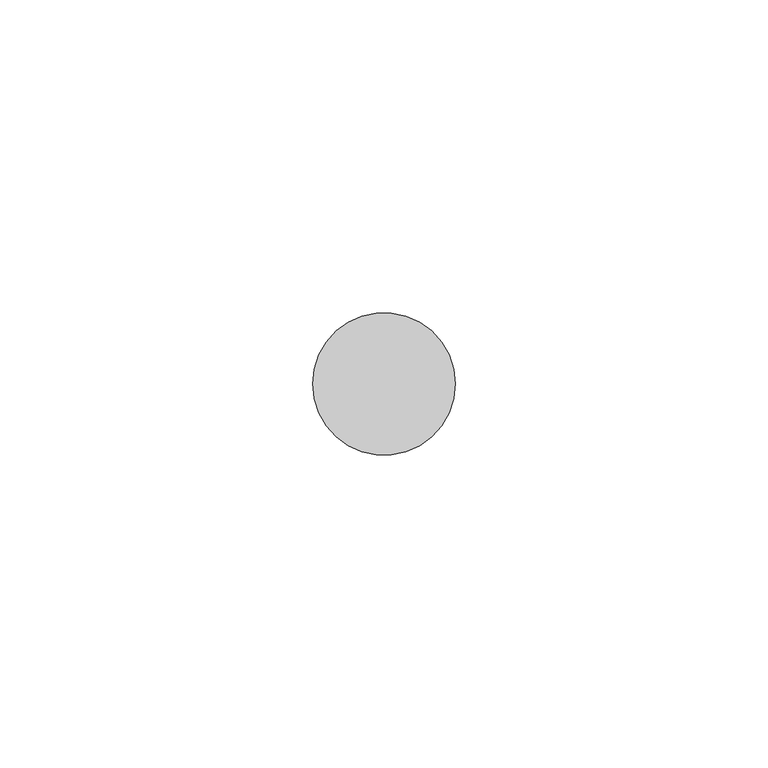
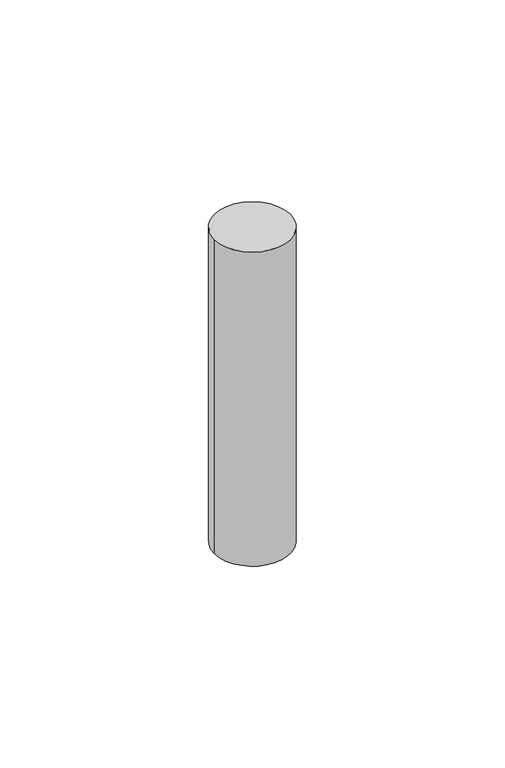
"""IFC4 building model written with IfcOpenShell, lengths in millimetres: proxy geometry, Bolt7:Bolt003:302961 : Bolt7:Bolt003:302961."""

from ifc_helpers import new_model, si_unit, point, frame, frame_2d, origin, place, context, project, spatial, circle_curve, trimmed, segment, composite_curve, outline, extrude, source, transform, mapped, element, save


def generic_models_6c568443(model_context):
    return source(origin(), model_context, "Body", "SweptSolid", [
        extrude(outline(composite_curve([segment(trimmed(circle_curve(frame_2d((12192.2703385, -1503.5124296)), 11.4045168), [point((12180.8658216, -1503.5124296))], [point((12203.6748553, -1503.5124296))], False, "CARTESIAN"), True, "CONTINUOUS"), segment(trimmed(circle_curve(frame_2d((12192.2703385, -1503.5124296)), 11.4045168), [point((12203.6748553, -1503.5124296))], [point((12180.8658216, -1503.5124296))], False, "CARTESIAN"), True, "CONTINUOUS")], self_intersect=False)), frame((0.0, 0.0, 39994.0914664), z_axis=(0.0, 0.0, 1.0), x_axis=(1.0, 0.0, 0.0)), (0.0, 0.0, 1.0), 99.5545336),
    ])


if __name__ == "__main__":
    model = new_model("IFC4")
    model_context = context("Model", 3, world=origin())
    ifc_project = project(units=[si_unit("LENGTHUNIT", "METRE", prefix="MILLI")], contexts=[model_context])
    site = spatial("IfcSite", under=ifc_project)
    building = spatial("IfcBuilding", under=site)
    placement = place(None, origin())
    generic_models_shape = generic_models_6c568443(model_context)
    element("IfcBuildingElementProxy", 1, Name="Bolt7:Bolt003:302961 : Bolt7:Bolt003:302961", ObjectType="Bolt7:Bolt003:302961 : Bolt7:Bolt003:302961", at=placement, inside=building, context=model_context, shape_type="MappedRepresentation", body=[
        mapped(generic_models_shape, transform((0.0, 0.0, 0.0), x_axis=(1.0, 0.0, 0.0), y_axis=(0.0, 1.0, 0.0), z_axis=(0.0, 0.0, 1.0))),
    ])
    save(model, "model.ifc")

# Revit data of these elements
# Type "Bolt7:Bolt003:302961 : Bolt7:Bolt003:302961"
#   NameOverride = "Bolt7:Bolt003:302961"
#   ObjectTypeOverride = "Bolt7:Bolt003"
#   Reference = "Bolt003"
#   Category = "Generic Models"
#   Tag = "302961"
# Element 1 (IfcBuildingElementProxy, "Bolt7:Bolt003:302961 : Bolt7:Bolt003:302961")
#   Materials on its faces: "BOLTS CONCEALED BY FLOOR FINISH"
# Materials
#   "BOLTS CONCEALED BY FLOOR FINISH": class "Unassigned", colour RGB 128 128 128, transparency 0
